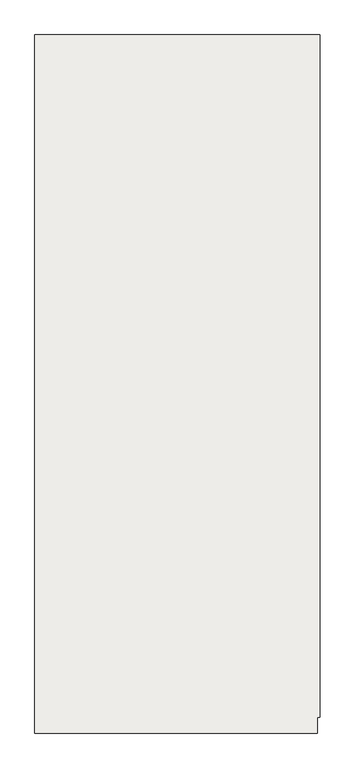
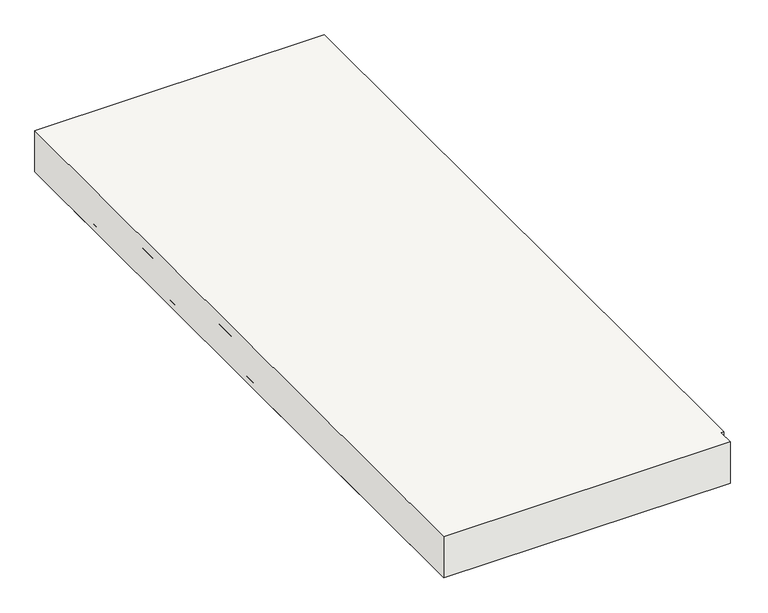
"""IFC4 building model written with IfcOpenShell, lengths in millimetres: slab geometry, Pano 6 (16 cm)."""

import ifcopenshell
import ifcopenshell.guid

model = None  # the IFC model being written
_history = None  # IfcOwnerHistory: only IFC2X3 demands one
_inside = {}  # id of a spatial element -> (the spatial element, [elements in it])
_under = {}  # id of a project, library or spatial element -> (it, [spatial elements below it])
_declared = {}  # id of a project -> (the project, [libraries it declares])
_typed = {}  # id of a type object -> (the type object, [elements of that type])
_made_of = {}  # id of a material, layer set ... -> (it, [elements and type objects made of it])


def new_model(schema):
    """Start an empty IFC model of exactly this schema.

    Asked for "IFC4X3", IfcOpenShell would pick the latest addendum, in which some entities
    have other attributes; the version numbers below select the first issue.
    IFC2X3 requires an IfcOwnerHistory on every rooted entity: one is made here for all.
    """
    global model, _history
    if schema == "IFC4X3":
        model = ifcopenshell.file(schema_version=(4, 3, 0, 0))
    else:
        model = ifcopenshell.file(schema=schema)
    _inside.clear()
    _under.clear()
    _declared.clear()
    _typed.clear()
    _made_of.clear()
    _history = None
    if model.schema == "IFC2X3":
        org = make("IfcOrganization", Name="unknown")
        user = make(
            "IfcPersonAndOrganization",
            ThePerson=make("IfcPerson", FamilyName="unknown"),
            TheOrganization=org,
        )
        app = make(
            "IfcApplication",
            ApplicationDeveloper=org,
            Version="unknown",
            ApplicationFullName="unknown",
            ApplicationIdentifier="unknown",
        )
        _history = make(
            "IfcOwnerHistory",
            OwningUser=user,
            OwningApplication=app,
            ChangeAction="ADDED",
            CreationDate=0,
        )
    return model


def make(cls, **values):
    """One entity of the class cls with the attributes given. An attribute that is None is left unset."""
    return model.create_entity(
        cls, **{name: value for name, value in values.items() if value is not None}
    )


def rooted(cls, **values):
    """An entity with a GlobalId (a new one), such as an element, a storey or a relation."""
    return make(cls, GlobalId=ifcopenshell.guid.new(), OwnerHistory=_history, **values)


def si_unit(unit_type, name, prefix=None):
    """IfcSIUnit, for example si_unit("LENGTHUNIT", "METRE", prefix="MILLI")."""
    return make("IfcSIUnit", UnitType=unit_type, Prefix=prefix, Name=name)


def assignment(units):
    """IfcUnitAssignment: the units of a project."""
    return None if units is None else make("IfcUnitAssignment", Units=units)


def point(xyz):
    """IfcCartesianPoint."""
    return None if xyz is None else make("IfcCartesianPoint", Coordinates=xyz)


def direction(xyz):
    """IfcDirection."""
    return None if xyz is None else make("IfcDirection", DirectionRatios=xyz)


def frame(location, z_axis=None, x_axis=None):
    """IfcAxis2Placement3D, a coordinate frame: its origin and axes. An axis left out is left unset."""
    return make(
        "IfcAxis2Placement3D",
        Location=point(location),
        Axis=direction(z_axis),
        RefDirection=direction(x_axis),
    )


def origin():
    """The frame at (0, 0, 0) with its axes left unset."""
    return frame((0.0, 0.0, 0.0))


def origin_with_axes():
    """The frame at (0, 0, 0) with the z axis (0, 0, 1) and the x axis (1, 0, 0) written out."""
    return frame((0.0, 0.0, 0.0), z_axis=(0.0, 0.0, 1.0), x_axis=(1.0, 0.0, 0.0))


def place(relative_to, where):
    """IfcLocalPlacement: puts the frame where relative to a parent placement (None: the world)."""
    return make(
        "IfcLocalPlacement", PlacementRelTo=relative_to, RelativePlacement=where
    )


def context(
    kind, dimensions, precision=None, world=None, true_north=None, identifier=None
):
    """IfcGeometricRepresentationContext, for example the 3D "Model" context."""
    return make(
        "IfcGeometricRepresentationContext",
        ContextIdentifier=identifier,
        ContextType=kind,
        CoordinateSpaceDimension=dimensions,
        Precision=precision,
        WorldCoordinateSystem=world,
        TrueNorth=true_north,
    )


def project(units=None, contexts=None):
    """IfcProject with its units and contexts."""
    return rooted(
        "IfcProject",
        Name="project",
        RepresentationContexts=contexts,
        UnitsInContext=assignment(units),
    )


def spatial(cls, under=None, at=None, **own):
    """A site, building, storey or space (cls), placed at a placement, below another one or the project."""
    s = rooted(cls, ObjectPlacement=at, **own)
    if under is not None:
        _under.setdefault(under.id(), (under, []))[1].append(s)
    return s


def polyline(points):
    """IfcPolyline through the points."""
    return make("IfcPolyline", Points=[point(p) for p in points])


def outline(outer, holes=None, kind="AREA"):
    """IfcArbitraryClosedProfileDef: a profile drawn as a closed curve; with holes, ...WithVoids."""
    if holes is None:
        return make("IfcArbitraryClosedProfileDef", ProfileType=kind, OuterCurve=outer)
    return make(
        "IfcArbitraryProfileDefWithVoids",
        ProfileType=kind,
        OuterCurve=outer,
        InnerCurves=holes,
    )


def extrude(swept, where, along, depth):
    """IfcExtrudedAreaSolid: the profile swept, set in the frame where, extruded along a direction by depth."""
    return make(
        "IfcExtrudedAreaSolid",
        SweptArea=swept,
        Position=where,
        ExtrudedDirection=direction(along),
        Depth=depth,
    )


def shape(context_of_items, identifier, shape_type, items):
    """IfcShapeRepresentation: the items that make up one representation, for example the "Body"."""
    return make(
        "IfcShapeRepresentation",
        ContextOfItems=context_of_items,
        RepresentationIdentifier=identifier,
        RepresentationType=shape_type,
        Items=items,
    )


def source(mapping_origin, context_of_items, identifier, shape_type, items):
    """IfcRepresentationMap: a shape defined once, which mapped items show again and again."""
    return make(
        "IfcRepresentationMap",
        MappingOrigin=mapping_origin,
        MappedRepresentation=shape(context_of_items, identifier, shape_type, items),
    )


def transform(
    local_origin,
    x_axis=None,
    y_axis=None,
    z_axis=None,
    scale=None,
    scale2=None,
    scale3=None,
    uniform=True,
):
    """IfcCartesianTransformationOperator3D, or its non-uniform kind. x_axis, y_axis, z_axis: its Axis1, 2, 3."""
    if uniform:
        return make(
            "IfcCartesianTransformationOperator3D",
            Axis1=direction(x_axis),
            Axis2=direction(y_axis),
            LocalOrigin=point(local_origin),
            Scale=scale,
            Axis3=direction(z_axis),
        )
    return make(
        "IfcCartesianTransformationOperator3DnonUniform",
        Axis1=direction(x_axis),
        Axis2=direction(y_axis),
        LocalOrigin=point(local_origin),
        Scale=scale,
        Axis3=direction(z_axis),
        Scale2=scale2,
        Scale3=scale3,
    )


def mapped(mapping_source, mapping_target):
    """IfcMappedItem: shows the shape of a source again, moved by a transform."""
    return make(
        "IfcMappedItem", MappingSource=mapping_source, MappingTarget=mapping_target
    )


def made_of(thing, what):
    """Note that an element or type object is made of a material, layer set ...; save() writes the relation."""
    if what is not None:
        _made_of.setdefault(what.id(), (what, []))[1].append(thing)
    return thing


def element(
    cls,
    number,
    at=None,
    inside=None,
    cuts=None,
    type_object=None,
    material=None,
    context=None,
    identifier="Body",
    shape_type=None,
    held_by="IfcProductDefinitionShape",
    body=None,
    shapes=None,
    **own,
):
    """One element of the class cls, such as IfcWall. Its Tag is "e" and its number.

    at: its placement. inside: the storey or other place that contains it. cuts: it is an
    opening in that element (IfcRelVoidsElement). A single representation is given by context,
    identifier, shape_type and body (its items); several are given by shapes. held_by: the class
    of the entity that holds the representations. save() writes the other relations.
    """
    e = rooted(cls, Tag="e%d" % number, ObjectPlacement=at, **own)
    if body is not None:
        shapes = [shape(context, identifier, shape_type, body)]
    if shapes is not None:
        e.Representation = make(held_by, Representations=shapes)
    if inside is not None:
        _inside.setdefault(inside.id(), (inside, []))[1].append(e)
    if cuts is not None:
        rooted(
            "IfcRelVoidsElement", RelatingBuildingElement=cuts, RelatedOpeningElement=e
        )
    if type_object is not None:
        _typed.setdefault(type_object.id(), (type_object, []))[1].append(e)
    return made_of(e, material)


def aggregate(whole, parts):
    """IfcRelAggregates: a whole, such as a stair, and the parts it consists of."""
    return rooted("IfcRelAggregates", RelatingObject=whole, RelatedObjects=parts)


def save(model, path):
    """Write the relations noted so far, then the file.

    IfcRelAggregates (storeys below a building ...), IfcRelContainedInSpatialStructure (elements
    in a storey), IfcRelDefinesByType, IfcRelAssociatesMaterial and IfcRelDeclares: one each for
    every whole, place, type object, material and project.
    """
    for whole, parts in _under.values():
        aggregate(whole, parts)
    for where, things in _inside.values():
        rooted(
            "IfcRelContainedInSpatialStructure",
            RelatedElements=things,
            RelatingStructure=where,
        )
    for kind, things in _typed.values():
        rooted("IfcRelDefinesByType", RelatedObjects=things, RelatingType=kind)
    for what, things in _made_of.values():
        rooted("IfcRelAssociatesMaterial", RelatedObjects=things, RelatingMaterial=what)
    for by, libraries in _declared.values():
        rooted("IfcRelDeclares", RelatingContext=by, RelatedDefinitions=libraries)
    model.write(path)


def slab_3da1eb17(model_context):
    return source(origin(), model_context, "Body", "SweptSolid", [
        extrude(outline(polyline([(5760.0, 8095.0), (5760.0, 5550.0), (5750.0, 5550.0), (5750.0, 5490.0), (4695.0, 5490.0), (4695.0, 8095.0), (5760.0, 8095.0)])), origin_with_axes(), (0.0, 0.0, 1.0), 160.0),
        extrude(outline(polyline([(5195.0, 6344.0), (5195.0, 6704.0), (5690.0, 6704.0), (5690.0, 6344.0), (5195.0, 6344.0)])), origin_with_axes(), (0.0, 0.0, 1.0), 120.0),
        extrude(outline(polyline([(4695.0, 6204.0), (4695.0, 6344.0), (5760.0, 6344.0), (5760.0, 6204.0), (4695.0, 6204.0)])), origin_with_axes(), (0.0, 0.0, 1.0), 24.0),
        extrude(outline(polyline([(4695.0, 6844.0), (4695.0, 7204.0), (5190.0, 7204.0), (5190.0, 6844.0), (4695.0, 6844.0)])), origin_with_axes(), (0.0, 0.0, 1.0), 120.0),
        extrude(outline(polyline([(4695.0, 5844.0), (4695.0, 6204.0), (5190.0, 6204.0), (5190.0, 5844.0), (4695.0, 5844.0)])), origin_with_axes(), (0.0, 0.0, 1.0), 120.0),
        extrude(outline(polyline([(4695.0, 6704.0), (4695.0, 6844.0), (5760.0, 6844.0), (5760.0, 6704.0), (4695.0, 6704.0)])), origin_with_axes(), (0.0, 0.0, 1.0), 24.0),
        extrude(outline(polyline([(5195.0, 5844.0), (5195.0, 6204.0), (5690.0, 6204.0), (5690.0, 5844.0), (5195.0, 5844.0)])), origin_with_axes(), (0.0, 0.0, 1.0), 120.0),
        extrude(outline(polyline([(5195.0, 7344.0), (5195.0, 7704.0), (5690.0, 7704.0), (5690.0, 7344.0), (5195.0, 7344.0)])), origin_with_axes(), (0.0, 0.0, 1.0), 120.0),
        extrude(outline(polyline([(4695.0, 6344.0), (4695.0, 6704.0), (5190.0, 6704.0), (5190.0, 6344.0), (4695.0, 6344.0)])), origin_with_axes(), (0.0, 0.0, 1.0), 120.0),
        extrude(outline(polyline([(5695.0, 5844.0), (5695.0, 6204.0), (5755.0, 6204.0), (5755.0, 5844.0), (5695.0, 5844.0)])), origin_with_axes(), (0.0, 0.0, 1.0), 120.0),
        extrude(outline(polyline([(5695.0, 7344.0), (5695.0, 7704.0), (5755.0, 7704.0), (5755.0, 7344.0), (5695.0, 7344.0)])), origin_with_axes(), (0.0, 0.0, 1.0), 120.0),
        extrude(outline(polyline([(5195.0, 6844.0), (5195.0, 7204.0), (5690.0, 7204.0), (5690.0, 6844.0), (5195.0, 6844.0)])), origin_with_axes(), (0.0, 0.0, 1.0), 120.0),
        extrude(outline(polyline([(4695.0, 5704.0), (4695.0, 5844.0), (5760.0, 5844.0), (5760.0, 5704.0), (4695.0, 5704.0)])), origin_with_axes(), (0.0, 0.0, 1.0), 24.0),
        extrude(outline(polyline([(4695.0, 7704.0), (4695.0, 7844.0), (5760.0, 7844.0), (5760.0, 7704.0), (4695.0, 7704.0)])), origin_with_axes(), (0.0, 0.0, 1.0), 24.0),
        extrude(outline(polyline([(5695.0, 6344.0), (5695.0, 6704.0), (5755.0, 6704.0), (5755.0, 6344.0), (5695.0, 6344.0)])), origin_with_axes(), (0.0, 0.0, 1.0), 120.0),
        extrude(outline(polyline([(4695.0, 7344.0), (4695.0, 7704.0), (5190.0, 7704.0), (5190.0, 7344.0), (4695.0, 7344.0)])), origin_with_axes(), (0.0, 0.0, 1.0), 120.0),
        extrude(outline(polyline([(4695.0, 7204.0), (4695.0, 7344.0), (5760.0, 7344.0), (5760.0, 7204.0), (4695.0, 7204.0)])), origin_with_axes(), (0.0, 0.0, 1.0), 24.0),
        extrude(outline(polyline([(5695.0, 6844.0), (5695.0, 7204.0), (5755.0, 7204.0), (5755.0, 6844.0), (5695.0, 6844.0)])), origin_with_axes(), (0.0, 0.0, 1.0), 120.0),
    ])


if __name__ == "__main__":
    model = new_model("IFC4")
    model_context = context("Model", 3, world=origin())
    ifc_project = project(units=[si_unit("LENGTHUNIT", "METRE", prefix="MILLI")], contexts=[model_context])
    site = spatial("IfcSite", under=ifc_project)
    building = spatial("IfcBuilding", under=site)
    placement = place(None, origin())
    slab_shape = slab_3da1eb17(model_context)
    element("IfcSlab", 1, ObjectType="Pano 6 (16 cm)", at=placement, inside=building, context=model_context, shape_type="MappedRepresentation", body=[
        mapped(slab_shape, transform((0.0, 0.0, 0.0), x_axis=(1.0, 0.0, 0.0), y_axis=(0.0, 1.0, 0.0), z_axis=(0.0, 0.0, 1.0))),
    ])
    save(model, "model.ifc")

# Revit data of these elements
# Element 1 (IfcSlab, "Pano 6 (16 cm)")
#   Materials on its faces: "Molde de poliestireno", "Concreto armado", "RGB 168-169-158"
# Materials
#   "Molde de poliestireno": class "Não atribuído", colour RGB 255 255 255, transparency 0
#   "Concreto armado": class "Não atribuído", colour RGB 168 169 158, transparency 0
#   "RGB 168-169-158": class "Não atribuído", colour RGB 168 169 158, transparency 0
